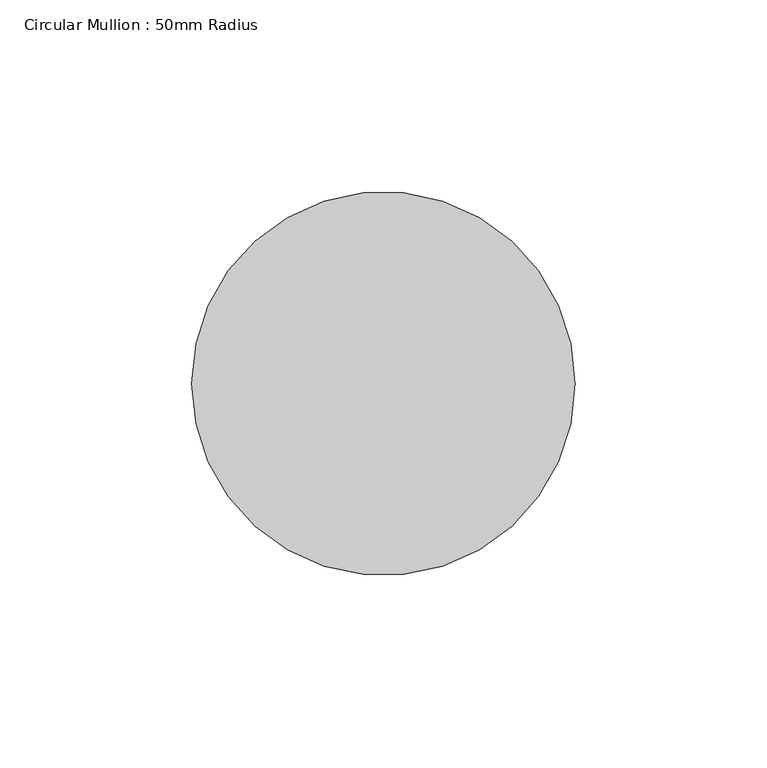
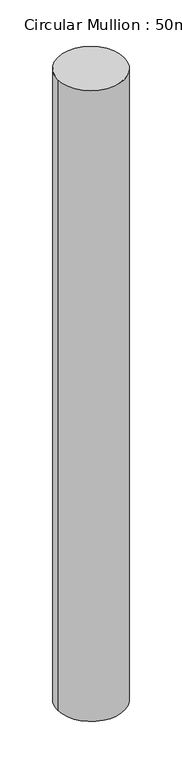
"""IFC4 building model written with IfcOpenShell, lengths in millimetres: member geometry, Circular Mullion : 50mm Radius."""

from ifc_helpers import new_model, si_unit, point, frame, origin, origin_2d, place, context, project, spatial, circle_curve, trimmed, segment, composite_curve, outline, extrude, source, transform, mapped, element, save


def circular_mullion_50mm_radius_8b02d008(model_context):
    return source(origin(), model_context, "Body", "SweptSolid", [
        extrude(outline(composite_curve([segment(trimmed(circle_curve(origin_2d(), 50.0), [point((50.0, 0.0))], [point((-50.0, 0.0))], False, "CARTESIAN"), True, "CONTINUOUS"), segment(trimmed(circle_curve(origin_2d(), 50.0), [point((-50.0, 0.0))], [point((50.0, 0.0))], False, "CARTESIAN"), True, "CONTINUOUS")], self_intersect=False)), frame((0.0, 0.0, -1002.0314253), z_axis=(0.0, 0.0, 1.0), x_axis=(1.0, 0.0, 0.0)), (0.0, 0.0, 1.0), 1002.0314253),
    ])


if __name__ == "__main__":
    model = new_model("IFC4")
    model_context = context("Model", 3, world=origin())
    ifc_project = project(units=[si_unit("LENGTHUNIT", "METRE", prefix="MILLI")], contexts=[model_context])
    site = spatial("IfcSite", under=ifc_project)
    building = spatial("IfcBuilding", under=site)
    placement = place(None, origin())
    circular_mullion_50mm_radius_shape = circular_mullion_50mm_radius_8b02d008(model_context)
    element("IfcMember", 1, ObjectType="Circular Mullion : 50mm Radius", at=placement, inside=building, context=model_context, shape_type="MappedRepresentation", body=[
        mapped(circular_mullion_50mm_radius_shape, transform((0.0, 0.0, 0.0), x_axis=(1.0, 0.0, 0.0), y_axis=(0.0, 1.0, 0.0), z_axis=(0.0, 0.0, 1.0))),
    ])
    save(model, "model.ifc")

# Revit data of these elements
# Type "Circular Mullion : 50mm Radius"
#   built-in parameter 1007350 = 0.164042 (stored number, unit not read)
# Element 1 (IfcMember, "Circular Mullion : 50mm Radius")
#   Materials on its faces: "Aluminium"
# Materials
#   "Aluminium": class "Metal", colour RGB 247 247 247, transparency 0, Description = "Aluminium 6061", Cost = 0
